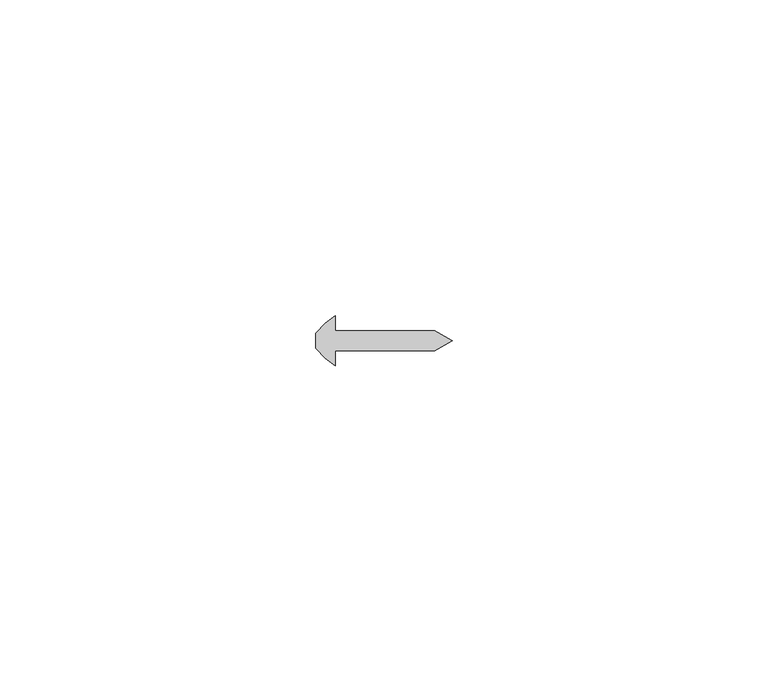
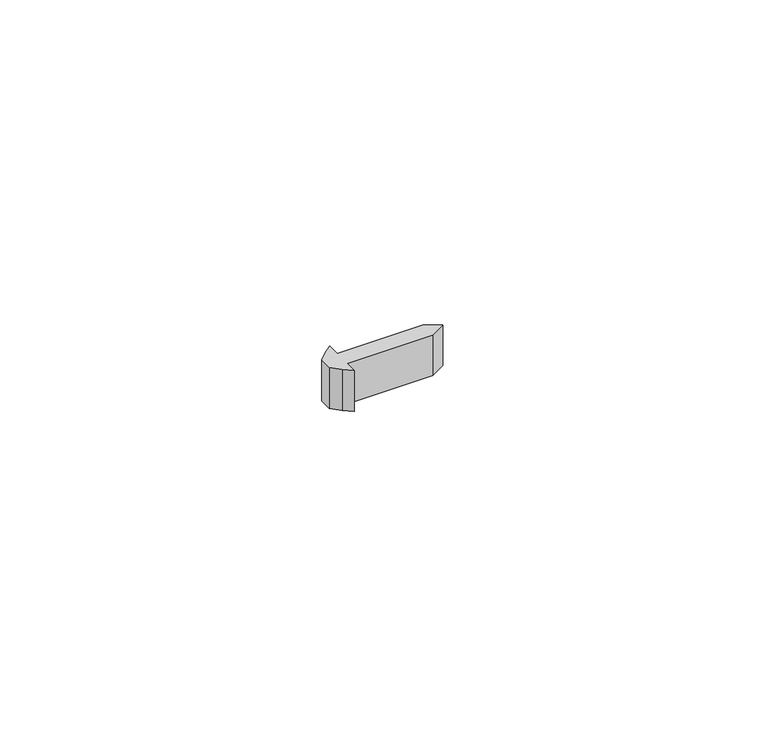
"""IFC4 building model written with IfcOpenShell, lengths in millimetres: proxy geometry, Generic Models 7:Generic Models 1:3:Generic Models 1:3 : Generic Models 7:Generic Models 1:305549:3:Generic Models 1:3:Generic Models 1:3 : Generic Models 7:Generic Models 1:305549:3 : Generic Models 7:Generic Models 1:3:Generic Models 1:3 : Generic Models 7:Generic Models 1:305549:301244:49 : Generic Models 7:Generic Models 1:3:Generic Models 1:3 : Generic Models 7:Generic Models 1:305549:3:Generic Models 1:3:Generic Models 1:3 : Generic Models 7:Generic Models 1:305549:3 : Generic Models 7:Generic Models 1:3:Generic Models 1:3 : Generic Models 7:Generic Models 1:305549:301244:308848."""

from ifc_helpers import new_model, si_unit, frame, origin, place, context, project, spatial, polyline, outline, extrude, source, transform, mapped, element, save


def generic_models_8a427471(model_context):
    return source(origin(), model_context, "Body", "SweptSolid", [
        extrude(outline(polyline([(560281.5242239, -578999.1038841), (560297.3334794, -578999.1038841), (560300.08311, -579000.6913841), (560297.3334794, -579002.2788841), (560281.5242239, -579002.2788841), (560281.5242239, -579004.6601341), (560279.9971659, -579003.4419385), (560278.4452757, -579001.8900483), (560278.4452757, -578999.4927198), (560279.9971659, -578997.9408296), (560281.5242239, -578996.7226341), (560281.5242239, -578999.1038841)])), frame((0.0, 0.0, 4907.75625), z_axis=(0.0, 0.0, 1.0), x_axis=(1.0, 0.0, 0.0)), (0.0, 0.0, 1.0), 7.9375),
    ])


if __name__ == "__main__":
    model = new_model("IFC4")
    model_context = context("Model", 3, world=origin())
    ifc_project = project(units=[si_unit("LENGTHUNIT", "METRE", prefix="MILLI")], contexts=[model_context])
    site = spatial("IfcSite", under=ifc_project)
    building = spatial("IfcBuilding", under=site)
    placement = place(None, origin())
    generic_models_shape = generic_models_8a427471(model_context)
    element("IfcBuildingElementProxy", 1, Name="Generic Models 7:Generic Models 1:3:Generic Models 1:3 : Generic Models 7:Generic Models 1:305549:3:Generic Models 1:3:Generic Models 1:3 : Generic Models 7:Generic Models 1:305549:3 : Generic Models 7:Generic Models 1:3:Generic Models 1:3 : Generic Models 7:Generic Models 1:305549:301244:49 : Generic Models 7:Generic Models 1:3:Generic Models 1:3 : Generic Models 7:Generic Models 1:305549:3:Generic Models 1:3:Generic Models 1:3 : Generic Models 7:Generic Models 1:305549:3 : Generic Models 7:Generic Models 1:3:Generic Models 1:3 : Generic Models 7:Generic Models 1:305549:301244:308848", ObjectType="Generic Models 7:Generic Models 1:3:Generic Models 1:3 : Generic Models 7:Generic Models 1:305549:3:Generic Models 1:3:Generic Models 1:3 : Generic Models 7:Generic Models 1:305549:3 : Generic Models 7:Generic Models 1:3:Generic Models 1:3 : Generic Models 7:Generic Models 1:305549:301244:49 : Generic Models 7:Generic Models 1:3:Generic Models 1:3 : Generic Models 7:Generic Models 1:305549:3:Generic Models 1:3:Generic Models 1:3 : Generic Models 7:Generic Models 1:305549:3 : Generic Models 7:Generic Models 1:3:Generic Models 1:3 : Generic Models 7:Generic Models 1:305549:301244:308848", at=placement, inside=building, context=model_context, shape_type="MappedRepresentation", body=[
        mapped(generic_models_shape, transform((0.0, 0.0, 0.0), x_axis=(1.0, 0.0, 0.0), y_axis=(0.0, 1.0, 0.0), z_axis=(0.0, 0.0, 1.0))),
    ])
    save(model, "model.ifc")

# Revit data of these elements
# Type "Generic Models 7:Generic Models 1:3:Generic Models 1:3 : Generic Models 7:Generic Models 1:305549:3:Generic Models 1:3:Generic Models 1:3 : Generic Models 7:Generic Models 1:305549:3 : Generic Models 7:Generic Models 1:3:Generic Models 1:3 : Generic Models 7:Generic Models 1:305549:301244:49 : Generic Models 7:Generic Models 1:3:Generic Models 1:3 : Generic Models 7:Generic Models 1:305549:3:Generic Models 1:3:Generic Models 1:3 : Generic Models 7:Generic Models 1:305549:3 : Generic Models 7:Generic Models 1:3:Generic Models 1:3 : Generic Models 7:Generic Models 1:305549:301244:308848"
#   NameOverride = "Generic Models 7:Generic Models 1:3:Generic Models 1:3 : Generic Models 7:Generic Models 1:305549:3:Generic Models 1:3:Generic Models 1:3 : Generic Models 7:Generic Models 1:305549:3 : Generic Models 7:Generic Models 1:3:Generic Models 1:3 : Generic Models 7:Generic Models 1:305549:301244:308848"
#   ObjectTypeOverride = "Generic Models 1:3:Generic Models 1:3 : Generic Models 7:Generic Models 1:305549:3 : Generic Models 7:Generic Models 1:3:Generic Models 1:3 : Generic Models 7:Generic Models 1:305549:301244"
#   Reference = "Generic Models 1"
#   Tag = "308848"
# Element 1 (IfcBuildingElementProxy, "Generic Models 7:Generic Models 1:3:Generic Models 1:3 : Generic Models 7:Generic Models 1:305549:3:Generic Models 1:3:Generic Models 1:3 : Generic Models 7:Generic Models 1:305549:3 : Generic Models 7:Generic Models 1:3:Generic Models 1:3 : Generic Models 7:Generic Models 1:305549:301244:49 : Generic Models 7:Generic Models 1:3:Generic Models 1:3 : Generic Models 7:Generic Models 1:305549:3:Generic Models 1:3:Generic Models 1:3 : Generic Models 7:Generic Models 1:305549:3 : Generic Models 7:Generic Models 1:3:Generic Models 1:3 : Generic Models 7:Generic Models 1:305549:301244:308848")
#   Materials on its faces: "FASTENERS (T.B.D)"
# Materials
#   "FASTENERS (T.B.D)": class "Generic", colour RGB 120 120 120, transparency 0, Cost = 0
